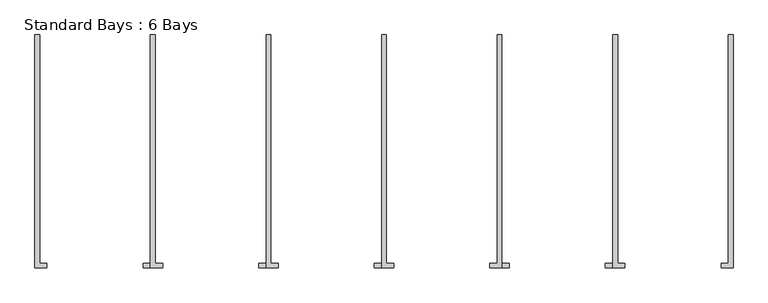
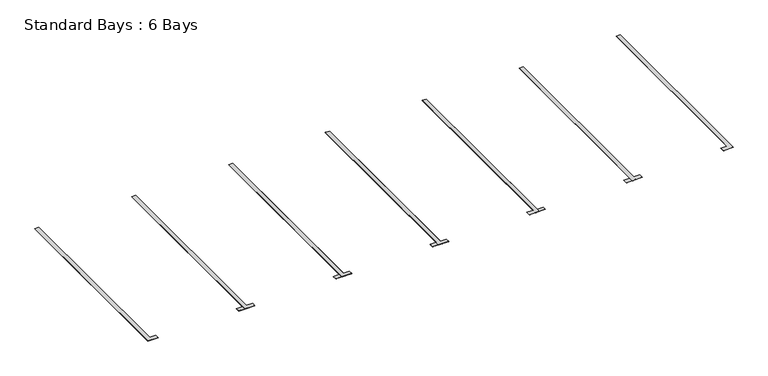
"""IFC4 building model written with IfcOpenShell, lengths in millimetres: proxy geometry, Standard Bays : 6 Bays."""

from ifc_helpers import new_model, si_unit, origin, origin_with_axes, place, context, project, spatial, polyline, outline, extrude, source, transform, mapped, element, save


def standard_bays_6_bays_a1d699d5(model_context):
    return source(origin(), model_context, "Body", "SweptSolid", [
        extrude(outline(polyline([(14350.0, 0.0), (14450.0, 0.0), (14450.0, -4850.0), (14200.0, -4850.0), (14200.0, -4750.0), (14350.0, -4750.0), (14350.0, 0.0)])), origin_with_axes(), (0.0, 0.0, 1.0), 3.175),
        extrude(outline(polyline([(11950.0, 0.0), (12050.0, 0.0), (12050.0, -4750.0), (12200.0, -4750.0), (12200.0, -4850.0), (11950.0, -4850.0), (11950.0, 0.0)])), origin_with_axes(), (0.0, 0.0, 1.0), 3.175),
        extrude(outline(polyline([(9550.0, 0.0), (9650.0, 0.0), (9650.0, -4850.0), (9400.0, -4850.0), (9400.0, -4750.0), (9550.0, -4750.0), (9550.0, 0.0)])), origin_with_axes(), (0.0, 0.0, 1.0), 3.175),
        extrude(outline(polyline([(7150.0, 0.0), (7250.0, 0.0), (7250.0, -4750.0), (7400.0, -4750.0), (7400.0, -4850.0), (7150.0, -4850.0), (7150.0, 0.0)])), origin_with_axes(), (0.0, 0.0, 1.0), 3.175),
        extrude(outline(polyline([(7150.0, 0.0), (7250.0, 0.0), (7250.0, -4850.0), (7000.0, -4850.0), (7000.0, -4750.0), (7150.0, -4750.0), (7150.0, 0.0)])), origin_with_axes(), (0.0, 0.0, 1.0), 3.175),
        extrude(outline(polyline([(4750.0, 0.0), (4850.0, 0.0), (4850.0, -4750.0), (5000.0, -4750.0), (5000.0, -4850.0), (4750.0, -4850.0), (4750.0, 0.0)])), origin_with_axes(), (0.0, 0.0, 1.0), 3.175),
        extrude(outline(polyline([(4750.0, 0.0), (4850.0, 0.0), (4850.0, -4850.0), (4600.0, -4850.0), (4600.0, -4750.0), (4750.0, -4750.0), (4750.0, 0.0)])), origin_with_axes(), (0.0, 0.0, 1.0), 3.175),
        extrude(outline(polyline([(2350.0, 0.0), (2450.0, 0.0), (2450.0, -4750.0), (2600.0, -4750.0), (2600.0, -4850.0), (2350.0, -4850.0), (2350.0, 0.0)])), origin_with_axes(), (0.0, 0.0, 1.0), 3.175),
        extrude(outline(polyline([(11950.0, 0.0), (12050.0, 0.0), (12050.0, -4850.0), (11800.0, -4850.0), (11800.0, -4750.0), (11950.0, -4750.0), (11950.0, 0.0)])), origin_with_axes(), (0.0, 0.0, 1.0), 3.175),
        extrude(outline(polyline([(9550.0, 0.0), (9650.0, 0.0), (9650.0, -4750.0), (9800.0, -4750.0), (9800.0, -4850.0), (9550.0, -4850.0), (9550.0, 0.0)])), origin_with_axes(), (0.0, 0.0, 1.0), 3.175),
        extrude(outline(polyline([(2350.0, 0.0), (2450.0, 0.0), (2450.0, -4850.0), (2200.0, -4850.0), (2200.0, -4750.0), (2350.0, -4750.0), (2350.0, 0.0)])), origin_with_axes(), (0.0, 0.0, 1.0), 3.175),
        extrude(outline(polyline([(-50.0, 0.0), (50.0, 0.0), (50.0, -4750.0), (200.0, -4750.0), (200.0, -4850.0), (-50.0, -4850.0), (-50.0, 0.0)])), origin_with_axes(), (0.0, 0.0, 1.0), 3.175),
    ])


if __name__ == "__main__":
    model = new_model("IFC4")
    model_context = context("Model", 3, world=origin())
    ifc_project = project(units=[si_unit("LENGTHUNIT", "METRE", prefix="MILLI")], contexts=[model_context])
    site = spatial("IfcSite", under=ifc_project)
    building = spatial("IfcBuilding", under=site)
    placement = place(None, origin())
    standard_bays_6_bays_shape = standard_bays_6_bays_a1d699d5(model_context)
    element("IfcBuildingElementProxy", 1, Name="Standard Bays : 6 Bays", ObjectType="Standard Bays : 6 Bays", at=placement, inside=building, context=model_context, shape_type="MappedRepresentation", body=[
        mapped(standard_bays_6_bays_shape, transform((0.0, 0.0, 0.0), x_axis=(1.0, 0.0, 0.0), y_axis=(0.0, 1.0, 0.0), z_axis=(0.0, 0.0, 1.0))),
    ])
    save(model, "model.ifc")

# Revit data of these elements
# Type "Standard Bays : 6 Bays"
#   Keynote = "Q22/185"
#   Length [instance default] = 14400 mm
#   Bay Width = 2400 mm
#   Bay Length = 4800 mm
#   No of Bays in Array [instance default] = 5
#   No of Bays [instance default] = 6
#   Material - White Lining = Paint - White Lining
# Element 1 (IfcBuildingElementProxy, "Standard Bays : 6 Bays")
#   Materials on its faces: "Paint - White Lining"
# Materials
#   "Paint - White Lining": class "Paint", colour RGB 239 247 247, transparency 0
